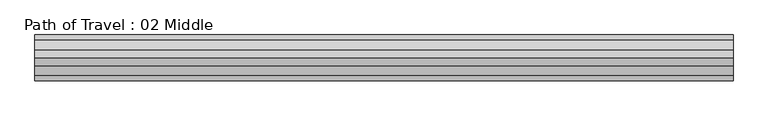
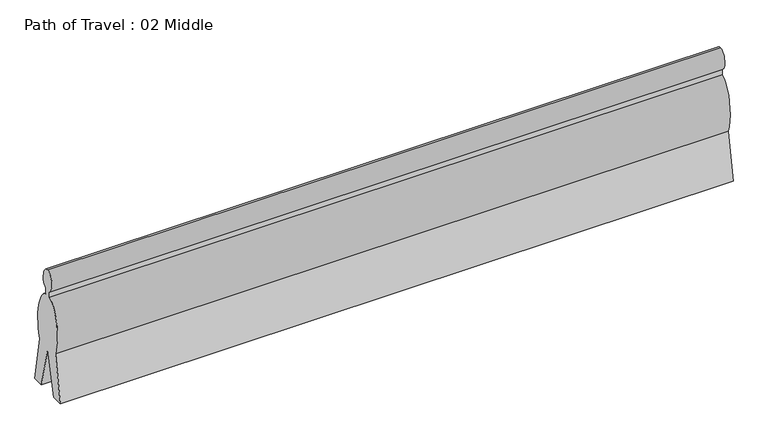
"""IFC4 building model written with IfcOpenShell, lengths in millimetres: proxy geometry, Path of Travel : 02 Middle."""

from ifc_helpers import new_model, si_unit, point, frame, origin, place, context, project, spatial, ellipse_curve, trimmed, source, transform, mapped, element, save
from ifc_brep_helpers import plane_surface, extruded_surface, advanced_brep


def path_of_travel_02_middle_e7c2b0a2(model_context):
    return source(origin(), model_context, "Body", "AdvancedBrep", [
        advanced_brep(
        [(227.5554837, 0.0, 1727.2), (227.5554837, 42.9018657, 1436.6534209), (227.5554837, 42.9018657, 1363.4763406), (227.5554837, 184.1186263, 643.4144547), (227.5554837, 297.5699544, 0.0), (227.5554837, 145.6574193, 0.0), (227.5554837, 0.0, 584.2), (227.5554837, -145.6574193, 0.0), (227.5554837, -297.5699544, 0.0), (227.5554837, -184.1186263, 643.4144547), (227.5554837, -42.9018657, 1363.4763406), (227.5554837, -42.9018657, 1436.6534209), (9301.1360347, 0.0, 1727.2), (9301.1360347, -42.9018657, 1436.6534209), (9301.1360347, -42.9018657, 1363.4763406), (9301.1360347, -184.1186263, 643.4144547), (9301.1360347, -297.5699544, 0.0), (9301.1360347, -145.6574193, 0.0), (9301.1360347, 0.0, 584.2), (9301.1360347, 145.6574193, 0.0), (9301.1360347, 297.5699544, 0.0), (9301.1360347, 184.1186263, 643.4144547), (9301.1360347, 42.9018657, 1363.4763406), (9301.1360347, 42.9018657, 1436.6534209)],
        [
            (0, 1, ellipse_curve(frame((227.5554837, 0.0, 1574.8), z_axis=(-1.0, 0.0, 0.0), x_axis=(0.0, 0.0, 1.0)), 152.4, 101.6)),
            (1, 2),
            (2, 3, ellipse_curve(frame((227.5554837, 0.0, 914.4), z_axis=(-1.0, 0.0, 0.0), x_axis=(0.0, 0.0, -1.0)), 457.2, 228.6)),
            (3, 4),
            (4, 5),
            (5, 6),
            (6, 7),
            (7, 8),
            (8, 9),
            (9, 10, ellipse_curve(frame((227.5554837, 0.0, 914.4), z_axis=(-1.0, 0.0, 0.0), x_axis=(0.0, 0.0, -1.0)), 457.2, 228.6)),
            (10, 11),
            (11, 0, ellipse_curve(frame((227.5554837, 0.0, 1574.8), z_axis=(-1.0, 0.0, 0.0), x_axis=(0.0, 0.0, 1.0)), 152.4, 101.6)),
            (12, 13, ellipse_curve(frame((9301.1360347, 0.0, 1574.8), z_axis=(1.0, 0.0, 0.0), x_axis=(0.0, 0.0, 1.0)), 152.4, 101.6)),
            (13, 14),
            (14, 15, ellipse_curve(frame((9301.1360347, 0.0, 914.4), z_axis=(1.0, 0.0, 0.0), x_axis=(0.0, 0.0, -1.0)), 457.2, 228.6)),
            (15, 16),
            (16, 17),
            (17, 18),
            (18, 19),
            (19, 20),
            (20, 21),
            (21, 22, ellipse_curve(frame((9301.1360347, 0.0, 914.4), z_axis=(1.0, 0.0, 0.0), x_axis=(0.0, 0.0, -1.0)), 457.2, 228.6)),
            (22, 23),
            (23, 12, ellipse_curve(frame((9301.1360347, 0.0, 1574.8), z_axis=(1.0, 0.0, 0.0), x_axis=(0.0, 0.0, 1.0)), 152.4, 101.6)),
            (0, 12),
            (23, 1),
            (22, 2),
            (21, 3),
            (20, 4),
            (19, 5),
            (18, 6),
            (17, 7),
            (16, 8),
            (15, 9),
            (14, 10),
            (13, 11),
        ],
        [
            plane_surface(frame((227.5554837, 0.0, 0.0), z_axis=(-1.0, 0.0, 0.0), x_axis=(0.0, 0.0, 1.0))),
            plane_surface(frame((9301.1360347, 0.0, 0.0), z_axis=(1.0, 0.0, 0.0), x_axis=(0.0, 0.0, 1.0))),
            extruded_surface(trimmed(ellipse_curve(frame((9301.1360347, 0.0, 1574.8), z_axis=(-1.0, 0.0, 0.0), x_axis=(0.0, 0.0, 1.0)), 152.4, 101.6), [point((9301.1360347, 0.0, 1727.2))], [point((9301.1360347, 42.9018657, 1436.6534209))], True, "CARTESIAN"), (-9073.580551000001, 0.0, 0.0), 9073.580551000001),
            plane_surface(frame((227.5554837, 42.9018657, 1436.6534209), z_axis=(0.0, 1.0, 0.0), x_axis=(1.0, 0.0, 0.0))),
            extruded_surface(trimmed(ellipse_curve(frame((9301.1360347, 0.0, 914.4), z_axis=(-1.0, 0.0, 0.0), x_axis=(0.0, 0.0, -1.0)), 457.2, 228.6), [point((9301.1360347, 42.9018657, 1363.4763406))], [point((9301.1360347, 184.1186263, 643.4144547))], True, "CARTESIAN"), (-9073.580551000001, 0.0, 0.0), 9073.580551000001),
            plane_surface(frame((227.5554837, 184.1186263, 643.4144547), z_axis=(0.0, 0.9848077530122078, 0.17364817766693205), x_axis=(1.0, 0.0, 0.0))),
            plane_surface(frame((227.5554837, 297.5699544, 0.0), z_axis=(0.0, 0.0, -1.0), x_axis=(1.0, 0.0, 0.0))),
            plane_surface(frame((227.5554837, 145.6574193, 0.0), z_axis=(0.0, -0.9702957262760199, -0.2419218955995739), x_axis=(1.0, 0.0, 0.0))),
            plane_surface(frame((227.5554837, 0.0, 584.2), z_axis=(0.0, 0.9702957262759961, -0.24192189559966923), x_axis=(1.0, 0.0, 0.0))),
            plane_surface(frame((227.5554837, -145.6574193, 0.0), z_axis=(0.0, 0.0, -1.0), x_axis=(1.0, 0.0, 0.0))),
            plane_surface(frame((227.5554837, -297.5699544, 0.0), z_axis=(0.0, -0.984807753012208, 0.17364817766693066), x_axis=(1.0, 0.0, 0.0))),
            extruded_surface(trimmed(ellipse_curve(frame((9301.1360347, 0.0, 914.4), z_axis=(-1.0, 0.0, 0.0), x_axis=(0.0, 0.0, -1.0)), 457.2, 228.6), [point((9301.1360347, -184.1186263, 643.4144547))], [point((9301.1360347, -42.9018657, 1363.4763406))], True, "CARTESIAN"), (-9073.580551000001, 0.0, 0.0), 9073.580551000001),
            plane_surface(frame((227.5554837, -42.9018657, 1363.4763406), z_axis=(0.0, -1.0, 0.0), x_axis=(1.0, 0.0, 0.0))),
            extruded_surface(trimmed(ellipse_curve(frame((9301.1360347, 0.0, 1574.8), z_axis=(-1.0, 0.0, 0.0), x_axis=(0.0, 0.0, 1.0)), 152.4, 101.6), [point((9301.1360347, -42.9018657, 1436.6534209))], [point((9301.1360347, 0.0, 1727.2))], True, "CARTESIAN"), (-9073.580551000001, 0.0, 0.0), 9073.580551000001),
        ],
        [
            (0, [[1, 2, 3, 4, 5, 6, 7, 8, 9, 10, 11, 12]]),
            (1, [[13, 14, 15, 16, 17, 18, 19, 20, 21, 22, 23, 24]]),
            (2, [[-1, 25, -24, 26]]),
            (3, [[-2, -26, -23, 27]]),
            (4, [[-3, -27, -22, 28]]),
            (5, [[-4, -28, -21, 29]]),
            (6, [[-5, -29, -20, 30]]),
            (7, [[-6, -30, -19, 31]]),
            (8, [[-7, -31, -18, 32]]),
            (9, [[-8, -32, -17, 33]]),
            (10, [[-9, -33, -16, 34]]),
            (11, [[-10, -34, -15, 35]]),
            (12, [[-11, -35, -14, 36]]),
            (13, [[-12, -36, -13, -25]]),
        ],
    ),
    ])


if __name__ == "__main__":
    model = new_model("IFC4")
    model_context = context("Model", 3, world=origin())
    ifc_project = project(units=[si_unit("LENGTHUNIT", "METRE", prefix="MILLI")], contexts=[model_context])
    site = spatial("IfcSite", under=ifc_project)
    building = spatial("IfcBuilding", under=site)
    placement = place(None, origin())
    path_of_travel_02_middle_shape = path_of_travel_02_middle_e7c2b0a2(model_context)
    element("IfcBuildingElementProxy", 1, Name="Path of Travel : 02 Middle", ObjectType="Path of Travel : 02 Middle", at=placement, inside=building, context=model_context, shape_type="MappedRepresentation", body=[
        mapped(path_of_travel_02_middle_shape, transform((0.0, 0.0, 0.0), x_axis=(1.0, 0.0, 0.0), y_axis=(0.0, 1.0, 0.0), z_axis=(0.0, 0.0, 1.0))),
    ])
    save(model, "model.ifc")

# Revit data of these elements
# Type "Path of Travel : 02 Middle"
#   Path of Egress [instance default] = 4' - 0"
#   built-in parameter 1001306 [instance default] = 4 (stored number, unit not read)
#   Dot at Start = no
#   Arrow in Middle = yes
#   Arrow at End = no
#   Egress Path = none
# Element 1 (IfcBuildingElementProxy, "Path of Travel : 02 Middle")
#   Path of Egress = 29' - 9.22758"
#   built-in parameter 1001306 = 29.769 (stored number, unit not read)
#   Materials on its faces: "Egress Path Solid"
# Materials
#   "Egress Path Solid": class "Unassigned", colour RGB 255 128 64, transparency 0.75, Comments = "Rendering appearance not upgraded "
